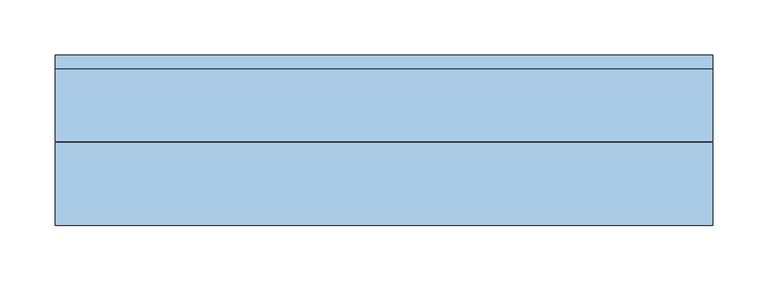
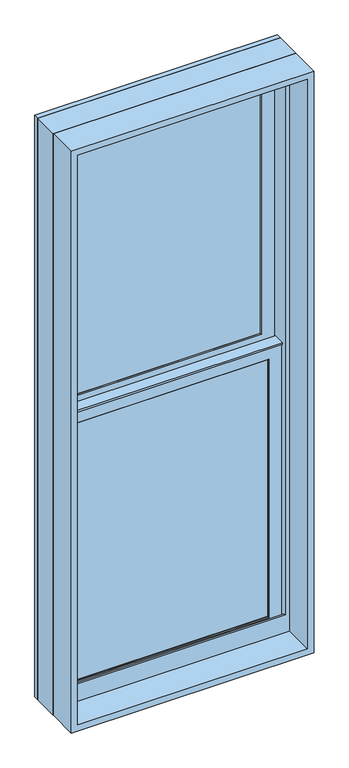
"""IFC4 building model written with IfcOpenShell, lengths in millimetres: window geometry, Window-Double_Hung-Marvin-Essential : ESDH2050."""

from ifc_helpers import new_model, si_unit, frame, origin, place, context, project, spatial, polyline, outline, extrude, faceted_brep, source, transform, mapped, element, save


def window_05ccaee4(model_context):
    return source(origin(), model_context, "Body", "SolidModel", [
        extrude(outline(polyline([(89.9583333, 20.6375), (89.9583333, 15.875), (70.9083333, 15.875), (70.9083333, 20.6375), (89.9583333, 20.6375)])), frame((0.0, 0.0, 984.25), z_axis=(0.0, 0.0, 1.0), x_axis=(1.0, 0.0, 0.0)), (0.0, 0.0, 1.0), 679.45),
        extrude(outline(polyline([(-70.9083333, 20.6375), (-70.9083333, 15.875), (-89.9583333, 15.875), (-89.9583333, 20.6375), (-70.9083333, 20.6375)])), frame((0.0, 0.0, 984.25), z_axis=(0.0, 0.0, 1.0), x_axis=(1.0, 0.0, 0.0)), (0.0, 0.0, 1.0), 679.45),
        extrude(outline(polyline([(241.3, 20.6375), (241.3, 15.875), (-241.3, 15.875), (-241.3, 20.6375), (241.3, 20.6375)])), frame((0.0, 0.0, 1314.45), z_axis=(0.0, 0.0, 1.0), x_axis=(1.0, 0.0, 0.0)), (0.0, 0.0, 1.0), 19.05),
        extrude(outline(polyline([(-89.9583333, 46.83125), (-89.9583333, 51.59375), (-70.9083333, 51.59375), (-70.9083333, 46.83125), (-89.9583333, 46.83125)])), frame((0.0, 0.0, 1701.8), z_axis=(0.0, 0.0, 1.0), x_axis=(1.0, 0.0, 0.0)), (0.0, 0.0, 1.0), 679.45),
        extrude(outline(polyline([(70.9083333, 46.83125), (70.9083333, 51.59375), (89.9583333, 51.59375), (89.9583333, 46.83125), (70.9083333, 46.83125)])), frame((0.0, 0.0, 1701.8), z_axis=(0.0, 0.0, 1.0), x_axis=(1.0, 0.0, 0.0)), (0.0, 0.0, 1.0), 679.45),
        extrude(outline(polyline([(-241.3, 46.83125), (-241.3, 51.59375), (241.3, 51.59375), (241.3, 46.83125), (-241.3, 46.83125)])), frame((0.0, 0.0, 2032.0), z_axis=(0.0, 0.0, 1.0), x_axis=(1.0, 0.0, 0.0)), (0.0, 0.0, 1.0), 19.05),
        extrude(outline(polyline([(89.9583333, 20.6375), (70.9083333, 20.6375), (70.9083333, 25.4), (89.9583333, 25.4), (89.9583333, 20.6375)])), frame((0.0, 0.0, 984.25), z_axis=(0.0, 0.0, 1.0), x_axis=(1.0, 0.0, 0.0)), (0.0, 0.0, 1.0), 679.45),
        extrude(outline(polyline([(-70.9083333, 20.6375), (-89.9583333, 20.6375), (-89.9583333, 25.4), (-70.9083333, 25.4), (-70.9083333, 20.6375)])), frame((0.0, 0.0, 984.25), z_axis=(0.0, 0.0, 1.0), x_axis=(1.0, 0.0, 0.0)), (0.0, 0.0, 1.0), 679.45),
        extrude(outline(polyline([(241.3, 20.6375), (-241.3, 20.6375), (-241.3, 25.4), (241.3, 25.4), (241.3, 20.6375)])), frame((0.0, 0.0, 1314.45), z_axis=(0.0, 0.0, 1.0), x_axis=(1.0, 0.0, 0.0)), (0.0, 0.0, 1.0), 19.05),
        extrude(outline(polyline([(-89.9583333, 56.35625), (-70.9083333, 56.35625), (-70.9083333, 51.59375), (-89.9583333, 51.59375), (-89.9583333, 56.35625)])), frame((0.0, 0.0, 1701.8), z_axis=(0.0, 0.0, 1.0), x_axis=(1.0, 0.0, 0.0)), (0.0, 0.0, 1.0), 679.45),
        extrude(outline(polyline([(70.9083333, 56.35625), (89.9583333, 56.35625), (89.9583333, 51.59375), (70.9083333, 51.59375), (70.9083333, 56.35625)])), frame((0.0, 0.0, 1701.8), z_axis=(0.0, 0.0, 1.0), x_axis=(1.0, 0.0, 0.0)), (0.0, 0.0, 1.0), 679.45),
        extrude(outline(polyline([(-241.3, 56.35625), (241.3, 56.35625), (241.3, 51.59375), (-241.3, 51.59375), (-241.3, 56.35625)])), frame((0.0, 0.0, 2032.0), z_axis=(0.0, 0.0, 1.0), x_axis=(1.0, 0.0, 0.0)), (0.0, 0.0, 1.0), 19.05),
        faceted_brep([(-268.2875, 5.6780605, 1693.7351748), (-268.2875, 5.6780605, 1689.1), (268.2875, 5.6780605, 1689.1), (268.2875, 5.6780605, 1693.7351748), (-268.2875, 34.8118605, 1693.7351748), (268.2875, 34.8118605, 1693.7351748), (268.2875, 34.8118605, 1689.1), (-268.2875, 34.8118605, 1689.1), (-268.2875, 30.1625, 1689.1), (-268.2875, 30.1625, 957.2625), (-268.2875, 8.9241104, 957.2625), (-268.2875, 8.9241104, 1689.1), (268.2875, 8.9241104, 1689.1), (268.2875, 30.1625, 1689.1), (268.2875, 8.9241104, 957.2625), (268.2875, 30.1625, 957.2625), (-252.4034752, 11.90625, 1674.8034752), (-252.4034752, 30.1625, 1674.8034752), (252.4034752, 30.1625, 1674.8034752), (252.4034752, 11.90625, 1674.8034752), (-235.74375, 10.4662439, 1658.14375), (-235.74375, 11.90625, 1658.14375), (235.74375, 11.90625, 1658.14375), (235.74375, 10.4662439, 1658.14375), (237.2858834, 8.9241104, 1659.6858834), (-237.2858834, 8.9241104, 1659.6858834), (252.4034752, 30.1625, 973.1465248), (252.4034752, 11.90625, 973.1465248), (235.74375, 11.90625, 989.80625), (235.74375, 10.4662439, 989.80625), (237.2858834, 8.9241104, 988.2641166), (-252.4034752, 30.1625, 973.1465248), (-252.4034752, 11.90625, 973.1465248), (-235.74375, 11.90625, 989.80625), (-235.74375, 10.4662439, 989.80625), (-237.2858834, 8.9241104, 988.2641166)], [[[0, 1, 2, 3]], [[4, 5, 6, 7]], [[1, 0, 4, 7, 8, 9, 10, 11]], [[2, 1, 11, 12]], [[7, 6, 13, 8]], [[3, 2, 12, 14, 15, 13, 6, 5]], [[0, 3, 5, 4]], [[16, 17, 18, 19]], [[20, 21, 22, 23]], [[20, 23, 24, 25]], [[19, 18, 26, 27]], [[23, 22, 28, 29]], [[24, 23, 29, 30]], [[27, 26, 31, 32]], [[29, 28, 33, 34]], [[30, 29, 34, 35]], [[15, 14, 10, 9]], [[15, 9, 8, 13], [18, 17, 31, 26]], [[17, 16, 32, 31]], [[16, 19, 27, 32], [22, 21, 33, 28]], [[21, 20, 34, 33]], [[20, 25, 35, 34]], [[10, 14, 12, 11], [25, 24, 30, 35]]]),
        extrude(outline(polyline([(38.5955581, 1674.8125), (33.5778968, 1674.8125), (33.5778968, 1676.4), (39.9405976, 1676.4), (39.9405976, 1674.8125), (61.515625, 1674.8125), (47.6307501, 1671.4975159), (38.5955581, 1671.4975159), (38.5955581, 1674.8125)])), frame((-268.2875, 0.0, 0.0), z_axis=(1.0, 0.0, 0.0), x_axis=(0.0, 1.0, 0.0)), (0.0, 0.0, 1.0), 536.575),
        faceted_brep([(298.45, 0.0, 927.1), (298.45, 0.0, 2438.4), (-298.45, 0.0, 2438.4), (-298.45, 0.0, 927.1), (272.25625, 0.0, 988.21875), (-272.25625, 0.0, 988.21875), (-272.25625, 0.0, 2412.20625), (272.25625, 0.0, 2412.20625), (272.25625, 3.96875, 927.1), (-272.25625, 3.96875, 927.1), (-272.25625, 3.96875, 988.21875), (272.25625, 3.96875, 988.21875), (-298.45, 65.6828125, 927.1), (-272.25625, 65.6828125, 927.1), (272.25625, 65.6828125, 927.1), (298.45, 65.6828125, 927.1), (-298.45, 65.6828125, 2438.4), (298.45, 65.6828125, 2438.4), (272.25625, 65.6828125, 2412.20625), (-272.25625, 65.6828125, 2412.20625)], [[[0, 1, 2, 3], [4, 5, 6, 7]], [[8, 9, 10, 11]], [[5, 4, 11, 10]], [[0, 3, 12, 13, 9, 8, 14, 15]], [[13, 12, 16, 17, 15, 14, 18, 19]], [[13, 19, 6, 5, 10, 9]], [[7, 6, 19, 18]], [[18, 14, 8, 11, 4, 7]], [[1, 0, 15, 17]], [[2, 1, 17, 16]], [[3, 2, 16, 12]]]),
        faceted_brep([(272.25625, 30.1625, 1682.75), (270.66875, 30.1625, 1682.75), (270.66875, 30.1625, 951.4544613), (272.25625, 30.1625, 951.4544613), (-270.66875, 30.1625, 1682.75), (-272.25625, 30.1625, 1682.75), (-272.25625, 30.1625, 951.4544613), (-270.66875, 30.1625, 951.4544613), (270.66875, 63.5, 1682.75), (272.25625, 63.5, 1682.75), (272.25625, 63.5, 944.9743077), (270.66875, 63.5, 944.9743077), (-272.25625, 63.5, 1682.75), (-270.66875, 63.5, 1682.75), (-270.66875, 63.5, 944.9743077), (-272.25625, 63.5, 944.9743077), (283.5108932, 3.96875, 956.5460105), (283.5108932, 3.96875, 927.1), (283.5108932, 65.6828125, 927.1), (283.5108932, 65.6828125, 944.550012), (-283.5108932, 3.96875, 927.1), (-283.5108932, 3.96875, 956.5460105), (-283.5108932, 65.6828125, 944.550012), (-283.5108932, 65.6828125, 927.1), (283.5108932, 78.58125, 942.0428097), (-283.5108932, 78.58125, 942.0428097), (-281.4971252, 68.2348864, 944.0539391), (-263.53135, 68.2348864, 944.0539391), (-263.53135, 65.6828125, 944.550012), (263.53135, 65.6828125, 944.550012), (263.53135, 68.2348864, 944.0539391), (281.4971252, 68.2348864, 944.0539391), (-298.45, 65.6828125, 927.1), (-298.45, 78.5948249, 927.1), (298.45, 78.5948249, 927.1), (298.45, 65.6828125, 927.1), (-298.45, 78.58125, 2438.4), (298.45, 78.58125, 2438.4), (283.5108932, 78.58125, 2423.4608932), (-283.5108932, 78.58125, 2423.4608932), (-298.45, 65.6828125, 2438.4), (-281.4971252, 68.2348864, 2421.4471252), (281.4971252, 68.2348864, 2421.4471252), (263.53135, 68.2348864, 2403.48135), (-263.53135, 68.2348864, 2403.48135), (-263.53135, 65.6828125, 2403.48135), (263.53135, 65.6828125, 2403.48135), (298.45, 65.6828125, 2438.4)], [[[0, 1, 2, 3]], [[4, 5, 6, 7]], [[8, 9, 10, 11]], [[12, 13, 14, 15]], [[1, 8, 11, 2]], [[9, 0, 3, 10]], [[1, 0, 9, 8]], [[5, 4, 13, 12]], [[5, 12, 15, 6]], [[13, 4, 7, 14]], [[16, 17, 18, 19]], [[20, 21, 22, 23]], [[24, 25, 26, 27, 28, 22, 21, 16, 19, 29, 30, 31], [3, 2, 11, 10], [7, 6, 15, 14]], [[17, 16, 21, 20]], [[17, 20, 23, 32, 33, 34, 35, 18]], [[34, 33, 36, 37], [25, 24, 38, 39]], [[33, 32, 40, 36]], [[39, 41, 26, 25]], [[41, 42, 31, 30, 43, 44, 27, 26]], [[44, 45, 28, 27]], [[40, 32, 23, 22, 28, 45, 46, 29, 19, 18, 35, 47]], [[36, 40, 47, 37]], [[39, 38, 42, 41]], [[44, 43, 46, 45]], [[34, 37, 47, 35]], [[42, 38, 24, 31]], [[46, 43, 30, 29]]]),
        extrude(outline(polyline([(248.44375, 11.90625), (-248.44375, 11.90625), (-248.44375, 15.08125), (248.44375, 15.08125), (248.44375, 11.90625)])), frame((0.0, 0.0, 977.10625), z_axis=(0.0, 0.0, 1.0), x_axis=(1.0, 0.0, 0.0)), (0.0, 0.0, 1.0), 693.7375),
        extrude(outline(polyline([(248.44375, 42.8625), (-248.44375, 42.8625), (-248.44375, 46.0375), (248.44375, 46.0375), (248.44375, 42.8625)])), frame((0.0, 0.0, 1694.65625), z_axis=(0.0, 0.0, 1.0), x_axis=(1.0, 0.0, 0.0)), (0.0, 0.0, 1.0), 693.7375),
        faceted_brep([(-235.74375, 31.194477, 1658.14375), (-237.2858834, 32.7366104, 1659.6858834), (237.2858834, 32.7366104, 1659.6858834), (235.74375, 31.194477, 1658.14375), (-235.74375, 30.1625, 1658.14375), (235.74375, 30.1625, 1658.14375), (-268.2875, 32.7366104, 1690.6875), (-268.2875, 30.1625, 1690.6875), (268.2875, 30.1625, 1690.6875), (268.2875, 32.7366104, 1690.6875), (237.2858834, 32.7366104, 988.2641166), (235.74375, 31.194477, 989.80625), (235.74375, 30.1625, 989.80625), (268.2875, 30.1625, 957.2625), (268.2875, 32.7366104, 957.2625), (-237.2858834, 32.7366104, 988.2641166), (-235.74375, 31.194477, 989.80625), (-235.74375, 30.1625, 989.80625), (-268.2875, 30.1625, 957.2625), (-268.2875, 32.7366104, 957.2625)], [[[0, 1, 2, 3]], [[4, 0, 3, 5]], [[6, 7, 8, 9]], [[3, 2, 10, 11]], [[5, 3, 11, 12]], [[9, 8, 13, 14]], [[11, 10, 15, 16]], [[12, 11, 16, 17]], [[14, 13, 18, 19]], [[9, 14, 19, 6], [1, 15, 10, 2]], [[16, 15, 1, 0]], [[17, 16, 0, 4]], [[7, 18, 13, 8], [5, 12, 17, 4]], [[19, 18, 7, 6]]]),
        faceted_brep([(-252.4034752, 42.8625, 2392.3534752), (-252.4034752, 61.11875, 2392.3534752), (252.4034752, 61.11875, 2392.3534752), (252.4034752, 42.8625, 2392.3534752), (-235.74375, 41.4224939, 2375.69375), (-235.74375, 42.8625, 2375.69375), (235.74375, 42.8625, 2375.69375), (235.74375, 41.4224939, 2375.69375), (-237.2858834, 39.8803604, 2377.2358834), (237.2858834, 39.8803604, 2377.2358834), (-268.2875, 61.11875, 2408.2375), (-268.2875, 39.8803604, 2408.2375), (268.2875, 39.8803604, 2408.2375), (268.2875, 61.11875, 2408.2375), (252.4034752, 61.11875, 1690.6965248), (252.4034752, 42.8625, 1690.6965248), (235.74375, 42.8625, 1707.35625), (235.74375, 41.4224939, 1707.35625), (237.2858834, 39.8803604, 1705.8141166), (268.2875, 39.8803604, 1674.8125), (268.2875, 61.11875, 1674.8125), (-252.4034752, 61.11875, 1690.6965248), (-252.4034752, 42.8625, 1690.6965248), (-235.74375, 42.8625, 1707.35625), (-235.74375, 41.4224939, 1707.35625), (-237.2858834, 39.8803604, 1705.8141166), (-268.2875, 39.8803604, 1674.8125), (-268.2875, 61.11875, 1674.8125)], [[[0, 1, 2, 3]], [[4, 5, 6, 7]], [[8, 4, 7, 9]], [[10, 11, 12, 13]], [[3, 2, 14, 15]], [[7, 6, 16, 17]], [[9, 7, 17, 18]], [[13, 12, 19, 20]], [[15, 14, 21, 22]], [[17, 16, 23, 24]], [[18, 17, 24, 25]], [[20, 19, 26, 27]], [[13, 20, 27, 10], [1, 21, 14, 2]], [[22, 21, 1, 0]], [[3, 15, 22, 0], [5, 23, 16, 6]], [[24, 23, 5, 4]], [[25, 24, 4, 8]], [[11, 26, 19, 12], [9, 18, 25, 8]], [[27, 26, 11, 10]]]),
        faceted_brep([(-268.2875, 61.11875, 1674.8125), (-268.2875, 63.6928604, 1674.8125), (268.2875, 63.6928604, 1674.8125), (268.2875, 61.11875, 1674.8125), (-235.74375, 62.150727, 1707.35625), (-235.74375, 61.11875, 1707.35625), (235.74375, 61.11875, 1707.35625), (235.74375, 62.150727, 1707.35625), (-237.2858834, 63.6928604, 1705.8141166), (237.2858834, 63.6928604, 1705.8141166), (268.2875, 63.6928604, 2408.2375), (268.2875, 61.11875, 2408.2375), (235.74375, 61.11875, 2375.69375), (235.74375, 62.150727, 2375.69375), (237.2858834, 63.6928604, 2377.2358834), (-268.2875, 63.6928604, 2408.2375), (-268.2875, 61.11875, 2408.2375), (-235.74375, 61.11875, 2375.69375), (-235.74375, 62.150727, 2375.69375), (-237.2858834, 63.6928604, 2377.2358834)], [[[0, 1, 2, 3]], [[4, 5, 6, 7]], [[8, 4, 7, 9]], [[3, 2, 10, 11]], [[7, 6, 12, 13]], [[9, 7, 13, 14]], [[11, 10, 15, 16]], [[13, 12, 17, 18]], [[14, 13, 18, 19]], [[16, 15, 1, 0]], [[3, 11, 16, 0], [5, 17, 12, 6]], [[18, 17, 5, 4]], [[19, 18, 4, 8]], [[1, 15, 10, 2], [9, 14, 19, 8]]]),
        extrude(outline(polyline([(248.44375, 26.19375), (-248.44375, 26.19375), (-248.44375, 30.1625), (248.44375, 30.1625), (248.44375, 26.19375)])), frame((0.0, 0.0, 977.10625), z_axis=(0.0, 0.0, 1.0), x_axis=(1.0, 0.0, 0.0)), (0.0, 0.0, 1.0), 693.7375),
        extrude(outline(polyline([(248.44375, 57.15), (-248.44375, 57.15), (-248.44375, 61.11875), (248.44375, 61.11875), (248.44375, 57.15)])), frame((0.0, 0.0, 1694.65625), z_axis=(0.0, 0.0, 1.0), x_axis=(1.0, 0.0, 0.0)), (0.0, 0.0, 1.0), 693.7375),
        extrude(outline(polyline([(2438.4, 298.45), (2438.4, -298.45), (927.1, -298.45), (927.1, 298.45), (2438.4, 298.45)]), holes=[polyline([(2422.525, 282.575), (942.975, 282.575), (942.975, -282.575), (2422.525, -282.575), (2422.525, 282.575)])]), frame((0.0, -76.2, 0.0), z_axis=(0.0, 1.0, 0.0), x_axis=(0.0, 0.0, 1.0)), (0.0, 0.0, 1.0), 75.40625),
    ])


if __name__ == "__main__":
    model = new_model("IFC4")
    model_context = context("Model", 3, world=origin())
    ifc_project = project(units=[si_unit("LENGTHUNIT", "METRE", prefix="MILLI")], contexts=[model_context])
    site = spatial("IfcSite", under=ifc_project)
    building = spatial("IfcBuilding", under=site)
    placement = place(None, origin())
    window_shape = window_05ccaee4(model_context)
    element("IfcWindow", 1, ObjectType="Window-Double_Hung-Marvin-Essential : ESDH2050", at=placement, inside=building, context=model_context, shape_type="MappedRepresentation", body=[
        mapped(window_shape, transform((0.0, 0.0, 0.0), x_axis=(1.0, 0.0, 0.0), y_axis=(0.0, 1.0, 0.0), z_axis=(0.0, 0.0, 1.0))),
    ])
    save(model, "model.ifc")

# Revit data of these elements
# Project information
#   Project Issue Date = "Issue Date"
#   Project Status = "Project Status"
#   Client Name = "Owner"
#   Project Address = "Enter address here"
#   Project Name = "Project Name"
#   Project Number = "Project Number"
# Type "Window-Double_Hung-Marvin-Essential : ESDH2050"
#   Type Mark = "62"
#   Window Type = "Essential Double Hung"
#   Product data url = "https://bimobject.com/marvin-windows-and-doors/product/marvin-dhwau"
#   Product Guid = "c4a96547-874c-4385-91dc-a058adc19d98"
#   Frame = "All Ultrex"
#   Egress Window = "No"
#   URL = "www.marvin.com"
#   Model = "ESDH2050"
#   Manufacturer = "Marvin Windows and Doors"
#   Label Egress = ""
#   Glass Type = "IG Low E II with Argon"
#   Design Pressure = "DP50"
#   Description = "2460 DBHG"
#   Analytic Construction = "<None>"
#   Prairie Corner Width = 0' - 4"
#   Prairie Corner Height = 0' - 4"
#   Egress Width = 1' - 8 9/16"
#   Egress Height = 2' - 1 27/128"
#   Rough Width = 2' - 0"
#   Rough Height = 5' - 0"
#   Nominal Width = 2' - 0"
#   Nominal Height = 5' - 0"
#   Inset to Installation Flange [instance default] = 0' - 1"
#   Height = 4' - 11 1/2"
#   Egress Area = 3.6 SF
#   Default Head Height = 8' - 0"
#   Width = 1' - 11 1/2"
#   Daylight Area = 6.78369 SF
#   DLO Width = 1' - 6 9/16"
#   DLO Height = 2' - 2 5/16"
#   Muntins Top Sash = yes
#   Lites Wide Top Sash = 3
#   Lites Wide Bottom Sash = 3
#   Lites High Top Sash = 2
#   Lites High Bottom Sash = 2
#   Lite Cut Prairie 9 = no
#   Lite Cut HV Grid = yes
#   Muntins Bottom Sash = yes
#   Label Visibility = no
#   Jamb Extension Visibility = yes
#   Edition number = 1
#   Interior Material = Ultrex-Marvin-Stonewhite
#   Glazing Material = Glass-Marvin-IG Low E II with Argon
#   Cladding Material = Ultrex-Marvin-Pebblegray
#   Wall Closure = (empty or 0)
#   Assembly Code = ""
# Element 1 (IfcWindow, "Window-Double_Hung-Marvin-Essential : ESDH2050")
#   Materials on its faces: "Ultrex-Marvin-Pebblegray", "Ultrex-Marvin-Stonewhite", "Glass-Marvin-IG Low E II with Argon"
# Materials
#   "Ultrex-Marvin-Stonewhite": class "Paint", colour RGB 250 251 245, transparency 0
#   "Glass-Marvin-IG Low E II with Argon": class "Glass", colour RGB 0 128 192, transparency 0.85
#   "Ultrex-Marvin-Pebblegray": class "Paint", colour RGB 189 185 173, transparency 0
